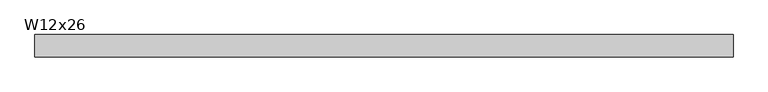
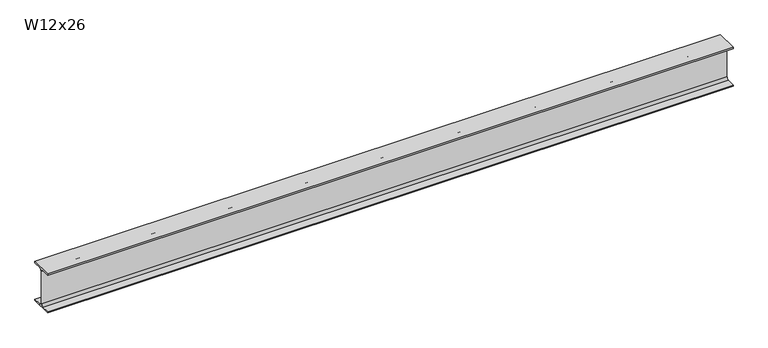
"""IFC4 building model written with IfcOpenShell, lengths in millimetres: beam geometry, RME W-Wide Flange : W12x26."""

from ifc_helpers import new_model, si_unit, point, frame, frame_2d, origin, place, context, project, spatial, polyline, circle_curve, trimmed, segment, composite_curve, outline, extrude, source, transform, mapped, element, save


def w12x26_5b2b7c56(model_context):
    return source(origin(), model_context, "Body", "SweptSolid", [
        extrude(outline(composite_curve([segment(polyline([(82.423, -145.288), (82.423, -154.94), (-82.423, -154.94), (-82.423, -145.288), (-20.2565, -145.288)]), True, "CONTINUOUS"), segment(trimmed(circle_curve(frame_2d((-20.2565, -127.9525)), 17.3355), [point((-20.2565, -145.288))], [point((-2.921, -127.9525))], True, "CARTESIAN"), True, "CONTINUOUS"), segment(polyline([(-2.921, -127.9525), (-2.921, 127.9525)]), True, "CONTINUOUS"), segment(trimmed(circle_curve(frame_2d((-20.2565, 127.9525)), 17.3355), [point((-2.921, 127.9525))], [point((-20.2565, 145.288))], True, "CARTESIAN"), True, "CONTINUOUS"), segment(polyline([(-20.2565, 145.288), (-82.423, 145.288), (-82.423, 154.94), (82.423, 154.94), (82.423, 145.288), (20.2565, 145.288)]), True, "CONTINUOUS"), segment(trimmed(circle_curve(frame_2d((20.2565, 127.9525)), 17.3355), [point((20.2565, 145.288))], [point((2.921, 127.9525))], True, "CARTESIAN"), True, "CONTINUOUS"), segment(polyline([(2.921, 127.9525), (2.921, -127.9525)]), True, "CONTINUOUS"), segment(trimmed(circle_curve(frame_2d((20.2565, -127.9525)), 17.3355), [point((2.921, -127.9525))], [point((20.2565, -145.288))], True, "CARTESIAN"), True, "CONTINUOUS"), segment(polyline([(20.2565, -145.288), (82.423, -145.288)]), True, "CONTINUOUS")], self_intersect=False)), frame((-2578.1, 0.0, 0.0), z_axis=(1.0, 0.0, 0.0), x_axis=(0.0, 1.0, 0.0)), (0.0, 0.0, 1.0), 5156.2),
    ])


if __name__ == "__main__":
    model = new_model("IFC4")
    model_context = context("Model", 3, world=origin())
    ifc_project = project(units=[si_unit("LENGTHUNIT", "METRE", prefix="MILLI")], contexts=[model_context])
    site = spatial("IfcSite", under=ifc_project)
    building = spatial("IfcBuilding", under=site)
    placement = place(None, origin())
    w12x26_shape = w12x26_5b2b7c56(model_context)
    element("IfcBeam", 1, ObjectType="RME W-Wide Flange : W12x26", at=placement, inside=building, context=model_context, shape_type="MappedRepresentation", body=[
        mapped(w12x26_shape, transform((0.0, 0.0, 0.0), x_axis=(1.0, 0.0, 0.0), y_axis=(0.0, 1.0, 0.0), z_axis=(0.0, 0.0, 1.0))),
    ])
    save(model, "model.ifc")

# Revit data of these elements
# Type "RME W-Wide Flange : W12x26"
#   WELD P [instance default] = ""
#   WELD LE [instance default] = ""
#   WELD D [instance default] = ""
#   TOP SECTION SIZE [instance default] = ""
#   TOP SECTION LENGTH [instance default] = ""
#   REMARKS [instance default] = ""
#   REINF TYPE [instance default] = ""
#   Nominal Size = "W24"
#   End Bearing Capacity [instance default] = ""
#   BOT SECTION SIZE [instance default] = ""
#   BOT SECTION LENGTH [instance default] = ""
#   Assembly Code = "B10"
#   W = 26
#   Start Extension Calculation [instance default] = 10' - 0"
#   Start Extension [instance default] = -0' - 0 1/2"
#   End Extension Calculation [instance default] = 10' - 0"
#   End Extension [instance default] = -0' - 0 1/2"
#   Length [instance default] = 5' - 0"
#   bf = 0' - 6.49"
#   d = 1' - 0.2"
#   k = 0' - 1 1/16"
#   k2 = 0' - 0.6825"
#   tf = 0' - 0.38"
#   tw = 0' - 0.23"
#   A = 0.053125 SF
#   Structural Material [instance default] = Metal - Steel - ASTM A992
# Element 1 (IfcBeam, "RME W-Wide Flange : W12x26")
#   Length = 16' - 11"
#   Materials on its faces: "Metal - Steel - ASTM A992"
# Materials
#   "Metal - Steel - ASTM A992": class "Metal", colour RGB 255 128 0, transparency 0
